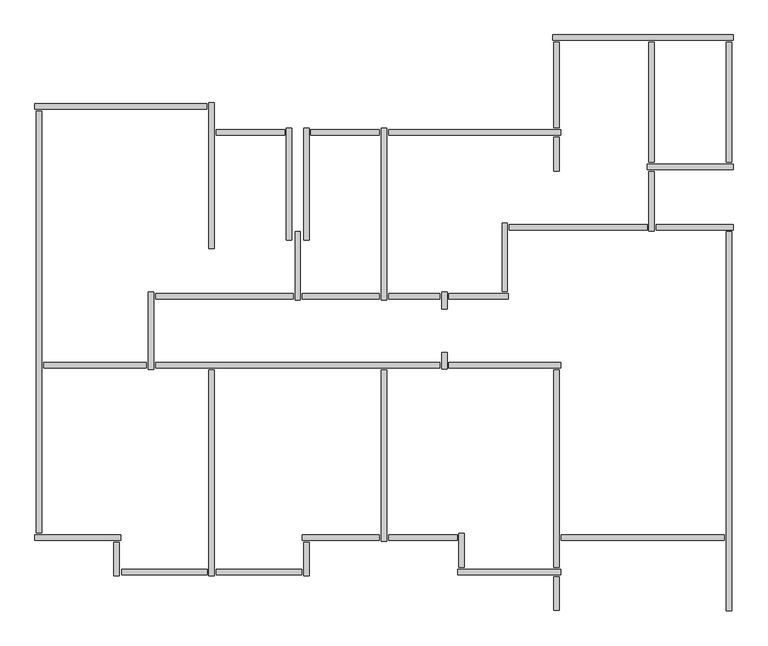
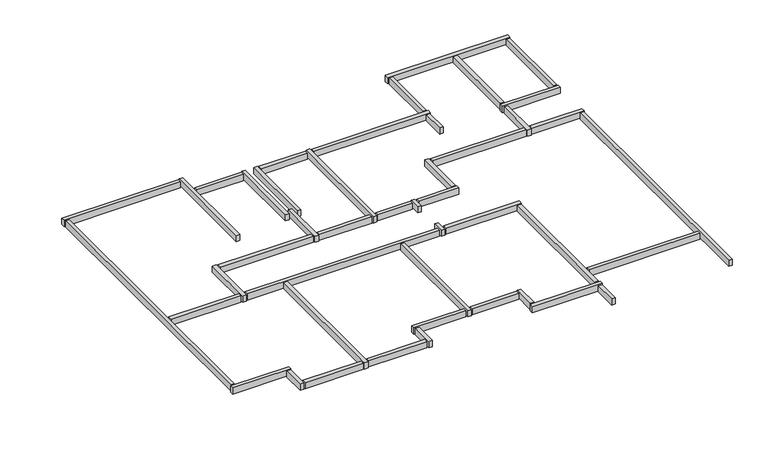
"""IFC4 building model written with IfcOpenShell, lengths in millimetres: beam geometry, Graute viga de respaldo14 : Graute viga de respaldo."""

from ifc_helpers import new_model, si_unit, frame, origin, place, context, project, spatial, polyline, outline, extrude, source, transform, mapped, element, save


def beam_e631fbc6(model_context):
    return source(origin(), model_context, "Body", "SweptSolid", [
        extrude(outline(polyline([(-75401.7587292, 57502.4278788), (-75401.7587292, 57408.4278788), (-76591.7587292, 57408.4278788), (-76591.7587292, 57502.4278788), (-75401.7587292, 57502.4278788)])), frame((0.0, 0.0, 11632.9999999), z_axis=(0.0, 0.0, 1.0), x_axis=(1.0, 0.0, 0.0)), (0.0, 0.0, 1.0), 167.0),
        extrude(outline(polyline([(-73751.7587292, 57502.4278788), (-73751.7587292, 57408.4278788), (-74941.7587292, 57408.4278788), (-74941.7587292, 57502.4278788), (-73751.7587292, 57502.4278788)])), frame((0.0, 0.0, 11632.9999999), z_axis=(0.0, 0.0, 1.0), x_axis=(1.0, 0.0, 0.0)), (0.0, 0.0, 1.0), 167.0),
        extrude(outline(polyline([(-77801.7587292, 53452.4278788), (-77801.7587292, 53358.4278788), (-79591.7587292, 53358.4278788), (-79591.7587292, 53452.4278788), (-77801.7587292, 53452.4278788)])), frame((0.0, 0.0, 11632.9999999), z_axis=(0.0, 0.0, 1.0), x_axis=(1.0, 0.0, 0.0)), (0.0, 0.0, 1.0), 167.0),
        extrude(outline(polyline([(-72401.7587292, 50452.4278788), (-72401.7587292, 50358.4278788), (-73591.7587292, 50358.4278788), (-73591.7587292, 50452.4278788), (-72401.7587292, 50452.4278788)])), frame((0.0, 0.0, 11632.9999999), z_axis=(0.0, 0.0, 1.0), x_axis=(1.0, 0.0, 0.0)), (0.0, 0.0, 1.0), 167.0),
        extrude(outline(polyline([(-72368.7587292, 50475.4278788), (-72274.7587292, 50475.4278788), (-72274.7587292, 49885.4278788), (-72368.7587292, 49885.4278788), (-72368.7587292, 50475.4278788)])), frame((0.0, 0.0, 11632.9999999), z_axis=(0.0, 0.0, 1.0), x_axis=(1.0, 0.0, 0.0)), (0.0, 0.0, 1.0), 167.0),
        extrude(outline(polyline([(-70601.7587292, 49852.4278788), (-70601.7587292, 49758.4278788), (-72391.7587292, 49758.4278788), (-72391.7587292, 49852.4278788), (-70601.7587292, 49852.4278788)])), frame((0.0, 0.0, 11632.9999999), z_axis=(0.0, 0.0, 1.0), x_axis=(1.0, 0.0, 0.0)), (0.0, 0.0, 1.0), 167.0),
        extrude(outline(polyline([(-72574.7587292, 53335.4278788), (-72668.7587292, 53335.4278788), (-72668.7587292, 53625.4278788), (-72574.7587292, 53625.4278788), (-72574.7587292, 53335.4278788)])), frame((0.0, 0.0, 11632.9999999), z_axis=(0.0, 0.0, 1.0), x_axis=(1.0, 0.0, 0.0)), (0.0, 0.0, 1.0), 167.0),
        extrude(outline(polyline([(-75251.7587292, 54652.4278788), (-75251.7587292, 54558.4278788), (-77641.7587292, 54558.4278788), (-77641.7587292, 54652.4278788), (-75251.7587292, 54652.4278788)])), frame((0.0, 0.0, 11632.9999999), z_axis=(0.0, 0.0, 1.0), x_axis=(1.0, 0.0, 0.0)), (0.0, 0.0, 1.0), 167.0),
        extrude(outline(polyline([(-73751.7587292, 54652.4278788), (-73751.7587292, 54558.4278788), (-75091.7587292, 54558.4278788), (-75091.7587292, 54652.4278788), (-73751.7587292, 54652.4278788)])), frame((0.0, 0.0, 11632.9999999), z_axis=(0.0, 0.0, 1.0), x_axis=(1.0, 0.0, 0.0)), (0.0, 0.0, 1.0), 167.0),
        extrude(outline(polyline([(-72701.7587292, 54652.4278788), (-72701.7587292, 54558.4278788), (-73591.7587292, 54558.4278788), (-73591.7587292, 54652.4278788), (-72701.7587292, 54652.4278788)])), frame((0.0, 0.0, 11632.9999999), z_axis=(0.0, 0.0, 1.0), x_axis=(1.0, 0.0, 0.0)), (0.0, 0.0, 1.0), 167.0),
        extrude(outline(polyline([(-72574.7587292, 54385.4278788), (-72668.7587292, 54385.4278788), (-72668.7587292, 54675.4278788), (-72574.7587292, 54675.4278788), (-72574.7587292, 54385.4278788)])), frame((0.0, 0.0, 11632.9999999), z_axis=(0.0, 0.0, 1.0), x_axis=(1.0, 0.0, 0.0)), (0.0, 0.0, 1.0), 167.0),
        extrude(outline(polyline([(-71511.7587292, 54652.4278788), (-71511.7587292, 54558.4278788), (-72541.7587292, 54558.4278788), (-72541.7587292, 54652.4278788), (-71511.7587292, 54652.4278788)])), frame((0.0, 0.0, 11632.9999999), z_axis=(0.0, 0.0, 1.0), x_axis=(1.0, 0.0, 0.0)), (0.0, 0.0, 1.0), 167.0),
        extrude(outline(polyline([(-71618.7587292, 55875.4278788), (-71524.7587292, 55875.4278788), (-71524.7587292, 54685.4278788), (-71618.7587292, 54685.4278788), (-71618.7587292, 55875.4278788)])), frame((0.0, 0.0, 11632.9999999), z_axis=(0.0, 0.0, 1.0), x_axis=(1.0, 0.0, 0.0)), (0.0, 0.0, 1.0), 167.0),
        extrude(outline(polyline([(-69091.7587292, 55852.4278788), (-69091.7587292, 55758.4278788), (-71491.7587292, 55758.4278788), (-71491.7587292, 55852.4278788), (-69091.7587292, 55852.4278788)])), frame((0.0, 0.0, 11632.9999999), z_axis=(0.0, 0.0, 1.0), x_axis=(1.0, 0.0, 0.0)), (0.0, 0.0, 1.0), 167.0),
        extrude(outline(polyline([(-73624.7587292, 54540.4278788), (-73718.7587292, 54540.4278788), (-73718.7587292, 57525.4278788), (-73624.7587292, 57525.4278788), (-73624.7587292, 54540.4278788)])), frame((0.0, 0.0, 11632.9999999), z_axis=(0.0, 0.0, 1.0), x_axis=(1.0, 0.0, 0.0)), (0.0, 0.0, 1.0), 167.0),
        extrude(outline(polyline([(-70601.7587292, 57502.4278788), (-70601.7587292, 57408.4278788), (-73591.7587292, 57408.4278788), (-73591.7587292, 57502.4278788), (-70601.7587292, 57502.4278788)])), frame((0.0, 0.0, 11632.9999999), z_axis=(0.0, 0.0, 1.0), x_axis=(1.0, 0.0, 0.0)), (0.0, 0.0, 1.0), 167.0),
        extrude(outline(polyline([(-70624.7587292, 56785.4278788), (-70718.7587292, 56785.4278788), (-70718.7587292, 57375.4278788), (-70624.7587292, 57375.4278788), (-70624.7587292, 56785.4278788)])), frame((0.0, 0.0, 11632.9999999), z_axis=(0.0, 0.0, 1.0), x_axis=(1.0, 0.0, 0.0)), (0.0, 0.0, 1.0), 167.0),
        extrude(outline(polyline([(-70718.7587292, 59025.4278788), (-70624.7587292, 59025.4278788), (-70624.7587292, 57535.4278788), (-70718.7587292, 57535.4278788), (-70718.7587292, 59025.4278788)])), frame((0.0, 0.0, 11632.9999999), z_axis=(0.0, 0.0, 1.0), x_axis=(1.0, 0.0, 0.0)), (0.0, 0.0, 1.0), 167.0),
        extrude(outline(polyline([(-67718.7587292, 59025.4278788), (-67624.7587292, 59025.4278788), (-67624.7587292, 56935.4278788), (-67718.7587292, 56935.4278788), (-67718.7587292, 59025.4278788)])), frame((0.0, 0.0, 11632.9999999), z_axis=(0.0, 0.0, 1.0), x_axis=(1.0, 0.0, 0.0)), (0.0, 0.0, 1.0), 167.0),
        extrude(outline(polyline([(-69068.7587292, 59025.4278788), (-68974.7587292, 59025.4278788), (-68974.7587292, 56935.4278788), (-69068.7587292, 56935.4278788), (-69068.7587292, 59025.4278788)])), frame((0.0, 0.0, 11632.9999999), z_axis=(0.0, 0.0, 1.0), x_axis=(1.0, 0.0, 0.0)), (0.0, 0.0, 1.0), 167.0),
        extrude(outline(polyline([(-68974.7587292, 55735.4278788), (-69068.7587292, 55735.4278788), (-69068.7587292, 56775.4278788), (-68974.7587292, 56775.4278788), (-68974.7587292, 55735.4278788)])), frame((0.0, 0.0, 11632.9999999), z_axis=(0.0, 0.0, 1.0), x_axis=(1.0, 0.0, 0.0)), (0.0, 0.0, 1.0), 167.0),
        extrude(outline(polyline([(-67751.7587292, 50452.4278788), (-67751.7587292, 50358.4278788), (-70591.7587292, 50358.4278788), (-70591.7587292, 50452.4278788), (-67751.7587292, 50452.4278788)])), frame((0.0, 0.0, 11632.9999999), z_axis=(0.0, 0.0, 1.0), x_axis=(1.0, 0.0, 0.0)), (0.0, 0.0, 1.0), 167.0),
        extrude(outline(polyline([(-70718.7587292, 53325.4278788), (-70624.7587292, 53325.4278788), (-70624.7587292, 49885.4278788), (-70718.7587292, 49885.4278788), (-70718.7587292, 53325.4278788)])), frame((0.0, 0.0, 11632.9999999), z_axis=(0.0, 0.0, 1.0), x_axis=(1.0, 0.0, 0.0)), (0.0, 0.0, 1.0), 167.0),
        extrude(outline(polyline([(-70601.7587292, 53452.4278788), (-70601.7587292, 53358.4278788), (-72541.7587292, 53358.4278788), (-72541.7587292, 53452.4278788), (-70601.7587292, 53452.4278788)])), frame((0.0, 0.0, 11632.9999999), z_axis=(0.0, 0.0, 1.0), x_axis=(1.0, 0.0, 0.0)), (0.0, 0.0, 1.0), 167.0),
        extrude(outline(polyline([(-72701.7587292, 53452.4278788), (-72701.7587292, 53358.4278788), (-77641.7587292, 53358.4278788), (-77641.7587292, 53452.4278788), (-72701.7587292, 53452.4278788)])), frame((0.0, 0.0, 11632.9999999), z_axis=(0.0, 0.0, 1.0), x_axis=(1.0, 0.0, 0.0)), (0.0, 0.0, 1.0), 167.0),
        extrude(outline(polyline([(-73624.7587292, 50335.4278788), (-73718.7587292, 50335.4278788), (-73718.7587292, 53325.4278788), (-73624.7587292, 53325.4278788), (-73624.7587292, 50335.4278788)])), frame((0.0, 0.0, 11632.9999999), z_axis=(0.0, 0.0, 1.0), x_axis=(1.0, 0.0, 0.0)), (0.0, 0.0, 1.0), 167.0),
        extrude(outline(polyline([(-75091.7587292, 50358.4278788), (-75091.7587292, 50452.4278788), (-73751.7587292, 50452.4278788), (-73751.7587292, 50358.4278788), (-75091.7587292, 50358.4278788)])), frame((0.0, 0.0, 11632.9999999), z_axis=(0.0, 0.0, 1.0), x_axis=(1.0, 0.0, 0.0)), (0.0, 0.0, 1.0), 167.0),
        extrude(outline(polyline([(-74974.7587292, 49735.4278788), (-75068.7587292, 49735.4278788), (-75068.7587292, 50325.4278788), (-74974.7587292, 50325.4278788), (-74974.7587292, 49735.4278788)])), frame((0.0, 0.0, 11632.9999999), z_axis=(0.0, 0.0, 1.0), x_axis=(1.0, 0.0, 0.0)), (0.0, 0.0, 1.0), 167.0),
        extrude(outline(polyline([(-75101.7587292, 49852.4278788), (-75101.7587292, 49758.4278788), (-76591.7587292, 49758.4278788), (-76591.7587292, 49852.4278788), (-75101.7587292, 49852.4278788)])), frame((0.0, 0.0, 11632.9999999), z_axis=(0.0, 0.0, 1.0), x_axis=(1.0, 0.0, 0.0)), (0.0, 0.0, 1.0), 167.0),
        extrude(outline(polyline([(-78230.736554, 49758.4278788), (-78230.736554, 49853.4278788), (-76741.7587292, 49853.4278788), (-76741.7587292, 49758.4278788), (-78230.736554, 49758.4278788)])), frame((0.0, 0.0, 11617.1856208), z_axis=(0.0, 0.0, 1.0), x_axis=(1.0, 0.0, 0.0)), (0.0, 0.0, 1.0), 165.0),
        extrude(outline(polyline([(-79718.7587292, 57825.4278788), (-79624.7587292, 57825.4278788), (-79624.7587292, 50485.4278788), (-79718.7587292, 50485.4278788), (-79718.7587292, 57825.4278788)])), frame((0.0, 0.0, 11632.9999999), z_axis=(0.0, 0.0, 1.0), x_axis=(1.0, 0.0, 0.0)), (0.0, 0.0, 1.0), 167.0),
        extrude(outline(polyline([(-77768.7587292, 54675.4278788), (-77674.7587292, 54675.4278788), (-77674.7587292, 53330.0746661), (-77768.7587292, 53330.0746661), (-77768.7587292, 54675.4278788)])), frame((0.0, 0.0, 11632.9999999), z_axis=(0.0, 0.0, 1.0), x_axis=(1.0, 0.0, 0.0)), (0.0, 0.0, 1.0), 167.0),
        extrude(outline(polyline([(-75218.7587292, 55725.4278788), (-75124.7587292, 55725.4278788), (-75124.7587292, 54535.4278788), (-75218.7587292, 54535.4278788), (-75218.7587292, 55725.4278788)])), frame((0.0, 0.0, 11632.9999999), z_axis=(0.0, 0.0, 1.0), x_axis=(1.0, 0.0, 0.0)), (0.0, 0.0, 1.0), 167.0),
        extrude(outline(polyline([(-75368.7587292, 57525.4278788), (-75274.7587292, 57525.4278788), (-75274.7587292, 55585.4278788), (-75368.7587292, 55585.4278788), (-75368.7587292, 57525.4278788)])), frame((0.0, 0.0, 11632.9999999), z_axis=(0.0, 0.0, 1.0), x_axis=(1.0, 0.0, 0.0)), (0.0, 0.0, 1.0), 167.0),
        extrude(outline(polyline([(-75068.7587292, 57525.4278788), (-74974.7587292, 57525.4278788), (-74974.7587292, 55585.4278788), (-75068.7587292, 55585.4278788), (-75068.7587292, 57525.4278788)])), frame((0.0, 0.0, 11632.9999999), z_axis=(0.0, 0.0, 1.0), x_axis=(1.0, 0.0, 0.0)), (0.0, 0.0, 1.0), 167.0),
        extrude(outline(polyline([(-76718.7587292, 57975.4278788), (-76624.7587292, 57975.4278788), (-76624.7587292, 55435.4278788), (-76718.7587292, 55435.4278788), (-76718.7587292, 57975.4278788)])), frame((0.0, 0.0, 11632.9999999), z_axis=(0.0, 0.0, 1.0), x_axis=(1.0, 0.0, 0.0)), (0.0, 0.0, 1.0), 167.0),
        extrude(outline(polyline([(-79741.7587292, 57858.4278788), (-79741.7587292, 57952.4278788), (-76751.7587292, 57952.4278788), (-76751.7587292, 57858.4278788), (-79741.7587292, 57858.4278788)])), frame((0.0, 0.0, 11632.9999999), z_axis=(0.0, 0.0, 1.0), x_axis=(1.0, 0.0, 0.0)), (0.0, 0.0, 1.0), 167.0),
        extrude(outline(polyline([(-78274.7587292, 49735.4278788), (-78368.7587292, 49735.4278788), (-78368.7587292, 50325.4278788), (-78274.7587292, 50325.4278788), (-78274.7587292, 49735.4278788)])), frame((0.0, 0.0, 11632.9999999), z_axis=(0.0, 0.0, 1.0), x_axis=(1.0, 0.0, 0.0)), (0.0, 0.0, 1.0), 167.0),
        extrude(outline(polyline([(-78251.7587292, 50452.4278788), (-78251.7587292, 50358.4278788), (-79741.7587292, 50358.4278788), (-79741.7587292, 50452.4278788), (-78251.7587292, 50452.4278788)])), frame((0.0, 0.0, 11632.9999999), z_axis=(0.0, 0.0, 1.0), x_axis=(1.0, 0.0, 0.0)), (0.0, 0.0, 1.0), 167.0),
        extrude(outline(polyline([(-76624.7587292, 49735.4278788), (-76718.7587292, 49735.4278788), (-76718.7587292, 53325.4278788), (-76624.7587292, 53325.4278788), (-76624.7587292, 49735.4278788)])), frame((0.0, 0.0, 11632.9999999), z_axis=(0.0, 0.0, 1.0), x_axis=(1.0, 0.0, 0.0)), (0.0, 0.0, 1.0), 167.0),
        extrude(outline(polyline([(-70624.7587292, 49135.4278788), (-70718.7587292, 49135.4278788), (-70718.7587292, 49725.4278788), (-70624.7587292, 49725.4278788), (-70624.7587292, 49135.4278788)])), frame((0.0, 0.0, 11632.9999999), z_axis=(0.0, 0.0, 1.0), x_axis=(1.0, 0.0, 0.0)), (0.0, 0.0, 1.0), 167.0),
        extrude(outline(polyline([(-67601.7587292, 56902.4278788), (-67601.7587292, 56808.4278788), (-69091.7587292, 56808.4278788), (-69091.7587292, 56902.4278788), (-67601.7587292, 56902.4278788)])), frame((0.0, 0.0, 11632.9999999), z_axis=(0.0, 0.0, 1.0), x_axis=(1.0, 0.0, 0.0)), (0.0, 0.0, 1.0), 167.0),
        extrude(outline(polyline([(-67601.7587292, 59152.4278788), (-67601.7587292, 59058.4278788), (-70741.7587292, 59058.4278788), (-70741.7587292, 59152.4278788), (-67601.7587292, 59152.4278788)])), frame((0.0, 0.0, 11632.9999999), z_axis=(0.0, 0.0, 1.0), x_axis=(1.0, 0.0, 0.0)), (0.0, 0.0, 1.0), 167.0),
        extrude(outline(polyline([(-67601.7587292, 55852.4278788), (-67601.7587292, 55758.4278788), (-68941.7587292, 55758.4278788), (-68941.7587292, 55852.4278788), (-67601.7587292, 55852.4278788)])), frame((0.0, 0.0, 11632.9999999), z_axis=(0.0, 0.0, 1.0), x_axis=(1.0, 0.0, 0.0)), (0.0, 0.0, 1.0), 167.0),
        extrude(outline(polyline([(-67624.7587292, 49132.8979841), (-67718.7587292, 49132.8979841), (-67718.7587292, 55725.4278788), (-67624.7587292, 55725.4278788), (-67624.7587292, 49132.8979841)])), frame((0.0, 0.0, 11632.9999999), z_axis=(0.0, 0.0, 1.0), x_axis=(1.0, 0.0, 0.0)), (0.0, 0.0, 1.0), 167.0),
    ])


if __name__ == "__main__":
    model = new_model("IFC4")
    model_context = context("Model", 3, world=origin())
    ifc_project = project(units=[si_unit("LENGTHUNIT", "METRE", prefix="MILLI")], contexts=[model_context])
    site = spatial("IfcSite", under=ifc_project)
    building = spatial("IfcBuilding", under=site)
    placement = place(None, origin())
    beam_shape = beam_e631fbc6(model_context)
    element("IfcBeam", 1, ObjectType="Graute viga de respaldo14 : Graute viga de respaldo", at=placement, inside=building, context=model_context, shape_type="MappedRepresentation", body=[
        mapped(beam_shape, transform((0.0, 0.0, 0.0), x_axis=(1.0, 0.0, 0.0), y_axis=(0.0, 1.0, 0.0), z_axis=(0.0, 0.0, 1.0))),
    ])
    save(model, "model.ifc")

# Revit data of these elements
# Element 1 (IfcBeam, "Graute viga de respaldo14 : Graute viga de respaldo")
#   Materials on its faces: "Concreto, Faixa de areia/cimento"
# Materials
#   "Concreto, Faixa de areia/cimento": class "Concreto", colour RGB 127 127 127, transparency 0, Description = "Revestimento de laje de concreto", Cost = 0
